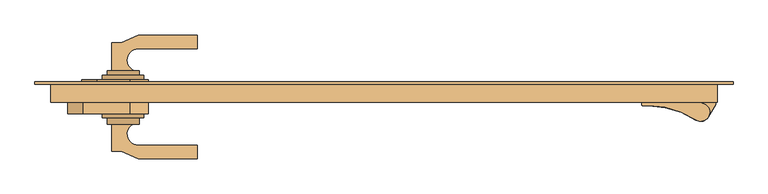
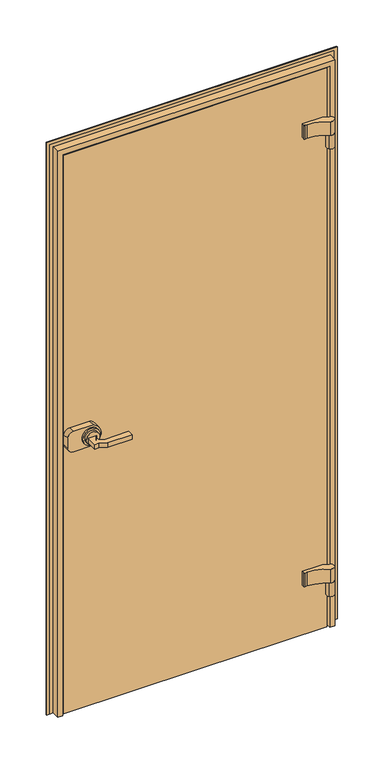
"""IFC4 building model written with IfcOpenShell, lengths in millimetres: door geometry, Doors_Doors_Faraone_Anta : Doors_Doors_Faraone_Anta."""

from ifc_helpers import new_model, si_unit, point, frame, frame_2d, origin, place, context, project, spatial, polyline, circle_curve, trimmed, segment, composite_curve, outline, extrude, faceted_brep, source, transform, mapped, element, save


def door_aa5b3e9e(model_context):
    return source(origin(), model_context, "Body", "SolidModel", [
        extrude(outline(polyline([(371.2008975, 11.599726), (440.9003723, 11.599726), (440.9003723, 1.8997991), (371.2008975, 1.8997991), (371.2008975, 11.599726)])), frame((0.0, 0.0, 1819.0000277), z_axis=(0.0, 0.0, 1.0), x_axis=(1.0, 0.0, 0.0)), (0.0, 0.0, 1.0), 50.0),
        extrude(outline(composite_curve([segment(polyline([(371.2008975, -17.600054), (371.2008975, -8.1001256), (441.2003701, -8.1001256), (441.2003701, -9.6001143), (460.8396194, -16.9560894)]), True, "CONTINUOUS"), segment(trimmed(circle_curve(frame_2d((456.200257, -29.0999673)), 12.9999021), [point((460.8396194, -16.9560894))], [point((449.4124725, -40.1870515))], False, "CARTESIAN"), True, "CONTINUOUS"), segment(trimmed(circle_curve(frame_2d((379.7862865, -147.5843675)), 127.9921454), [point((449.4124725, -40.1870515))], [point((381.2008221, -19.6000389))], True, "CARTESIAN"), True, "CONTINUOUS"), segment(polyline([(381.2008221, -19.6000389), (373.2008824, -19.6000389)]), True, "CONTINUOUS"), segment(trimmed(circle_curve(frame_2d((373.2008824, -17.600054)), 1.9999849), [point((373.2008824, -19.6000389))], [point((371.2008975, -17.600054))], False, "CARTESIAN"), True, "CONTINUOUS")], self_intersect=False)), frame((0.0, 0.0, 1819.0000277), z_axis=(0.0, 0.0, 1.0), x_axis=(1.0, 0.0, 0.0)), (0.0, 0.0, 1.0), 50.0),
        extrude(outline(composite_curve([segment(polyline([(478.0000928, -18.0609582), (467.2229983, -35.9917471)]), True, "CONTINUOUS"), segment(trimmed(circle_curve(frame_2d((456.200257, -29.0999673)), 12.9999021), [point((467.2229983, -35.9917471))], [point((445.8509495, -36.9669419))], False, "CARTESIAN"), True, "CONTINUOUS"), segment(trimmed(circle_curve(frame_2d((456.200257, -29.0999673)), 12.9999021), [point((445.8509495, -36.9669419))], [point((451.8171202, -16.861276))], False, "CARTESIAN"), True, "CONTINUOUS"), segment(polyline([(451.8171202, -16.861276), (456.2037355, -15.0000736), (478.0000928, -15.0000736), (478.0000928, -18.0609582)]), True, "CONTINUOUS")], self_intersect=False)), frame((0.0, 0.0, 1769.0000277), z_axis=(0.0, 0.0, 1.0), x_axis=(1.0, 0.0, 0.0)), (0.0, 0.0, 1.0), 50.0),
        extrude(outline(polyline([(371.2008975, 11.599726), (440.9003723, 11.599726), (440.9003723, 1.8997991), (371.2008975, 1.8997991), (371.2008975, 11.599726)])), frame((0.0, 0.0, 182.0), z_axis=(0.0, 0.0, 1.0), x_axis=(1.0, 0.0, 0.0)), (0.0, 0.0, 1.0), 50.0),
        extrude(outline(composite_curve([segment(polyline([(371.2008975, -17.600054), (371.2008975, -8.1001256), (441.2003701, -8.1001256), (441.2003701, -9.6001143), (460.8396194, -16.9560894)]), True, "CONTINUOUS"), segment(trimmed(circle_curve(frame_2d((456.200257, -29.0999673)), 12.9999021), [point((460.8396194, -16.9560894))], [point((449.4124725, -40.1870515))], False, "CARTESIAN"), True, "CONTINUOUS"), segment(trimmed(circle_curve(frame_2d((379.7862865, -147.5843675)), 127.9921454), [point((449.4124725, -40.1870515))], [point((381.2008221, -19.6000389))], True, "CARTESIAN"), True, "CONTINUOUS"), segment(polyline([(381.2008221, -19.6000389), (373.2008824, -19.6000389)]), True, "CONTINUOUS"), segment(trimmed(circle_curve(frame_2d((373.2008824, -17.600054)), 1.9999849), [point((373.2008824, -19.6000389))], [point((371.2008975, -17.600054))], False, "CARTESIAN"), True, "CONTINUOUS")], self_intersect=False)), frame((0.0, 0.0, 182.0), z_axis=(0.0, 0.0, 1.0), x_axis=(1.0, 0.0, 0.0)), (0.0, 0.0, 1.0), 50.0),
        extrude(outline(composite_curve([segment(polyline([(478.0000928, -18.0609582), (467.2229983, -35.9917471)]), True, "CONTINUOUS"), segment(trimmed(circle_curve(frame_2d((456.200257, -29.0999673)), 12.9999021), [point((467.2229983, -35.9917471))], [point((445.8509495, -36.9669419))], False, "CARTESIAN"), True, "CONTINUOUS"), segment(trimmed(circle_curve(frame_2d((456.200257, -29.0999673)), 12.9999021), [point((445.8509495, -36.9669419))], [point((451.8171202, -16.861276))], False, "CARTESIAN"), True, "CONTINUOUS"), segment(polyline([(451.8171202, -16.861276), (456.2037355, -15.0000736), (478.0000928, -15.0000736), (478.0000928, -18.0609582)]), True, "CONTINUOUS")], self_intersect=False)), frame((0.0, 0.0, 132.0), z_axis=(0.0, 0.0, 1.0), x_axis=(1.0, 0.0, 0.0)), (0.0, 0.0, 1.0), 50.0),
        extrude(outline(composite_curve([segment(trimmed(circle_curve(frame_2d((1003.2884985, -375.8959538)), 23.0897305), [point((1003.2884985, -398.9856843))], [point((1003.2884985, -352.8062233))], False, "CARTESIAN"), True, "CONTINUOUS"), segment(trimmed(circle_curve(frame_2d((1003.2884985, -375.8959538)), 23.0897305), [point((1003.2884985, -352.8062233))], [point((1003.2884985, -398.9856843))], False, "CARTESIAN"), True, "CONTINUOUS")], self_intersect=False)), frame((0.0, -46.355004, 0.0), z_axis=(0.0, 1.0, 0.0), x_axis=(0.0, 0.0, 1.0)), (0.0, 0.0, 1.0), 9.3686894),
        extrude(outline(composite_curve([segment(trimmed(circle_curve(frame_2d((987.7717852, -433.4834563)), 22.4105262), [point((983.5880679, -455.5))], [point((965.361259, -433.4834563))], False, "CARTESIAN"), True, "CONTINUOUS"), segment(polyline([(965.361259, -433.4834563), (965.361259, -368.4834563)]), True, "CONTINUOUS"), segment(trimmed(circle_curve(frame_2d((1002.861259, -378.1489886)), 38.7256054), [point((965.361259, -368.4834563))], [point((1039.5100566, -365.6374682))], False, "CARTESIAN"), True, "CONTINUOUS"), segment(polyline([(1039.5100566, -365.6374682), (1039.5100566, -433.4834563)]), True, "CONTINUOUS"), segment(trimmed(circle_curve(frame_2d((1017.0995304, -433.4834563)), 22.4105262), [point((1039.5100566, -433.4834563))], [point((1021.2832478, -455.5))], False, "CARTESIAN"), True, "CONTINUOUS"), segment(polyline([(1021.2832478, -455.5), (983.5880679, -455.5)]), True, "CONTINUOUS")], self_intersect=False)), frame((0.0, -31.1653283, 0.0), z_axis=(0.0, 1.0, 0.0), x_axis=(0.0, 0.0, 1.0)), (0.0, 0.0, 1.0), 23.0652027),
        extrude(outline(composite_curve([segment(trimmed(circle_curve(frame_2d((987.7717852, -433.4834563)), 22.4105262), [point((983.5880679, -455.5))], [point((965.361259, -433.4834563))], False, "CARTESIAN"), True, "CONTINUOUS"), segment(polyline([(965.361259, -433.4834563), (965.361259, -368.4834563)]), True, "CONTINUOUS"), segment(trimmed(circle_curve(frame_2d((1002.861259, -378.1489886)), 38.7256054), [point((965.361259, -368.4834563))], [point((1039.5100566, -365.6374682))], False, "CARTESIAN"), True, "CONTINUOUS"), segment(polyline([(1039.5100566, -365.6374682), (1039.5100566, -433.4834563)]), True, "CONTINUOUS"), segment(trimmed(circle_curve(frame_2d((1017.0995304, -433.4834563)), 22.4105262), [point((1039.5100566, -433.4834563))], [point((1021.2832478, -455.5))], False, "CARTESIAN"), True, "CONTINUOUS"), segment(polyline([(1021.2832478, -455.5), (983.5880679, -455.5)]), True, "CONTINUOUS")], self_intersect=False)), frame((0.0, -31.1653283, 0.0), z_axis=(0.0, 1.0, 0.0), x_axis=(0.0, 0.0, 1.0)), (0.0, 0.0, 1.0), 23.0652027),
        extrude(outline(composite_curve([segment(trimmed(circle_curve(frame_2d((1003.2884985, -375.8959538)), 30.0), [point((1003.2884985, -405.8959538))], [point((1003.2884985, -345.8959538))], False, "CARTESIAN"), True, "CONTINUOUS"), segment(trimmed(circle_curve(frame_2d((1003.2884985, -375.8959538)), 30.0), [point((1003.2884985, -345.8959538))], [point((1003.2884985, -405.8959538))], False, "CARTESIAN"), True, "CONTINUOUS")], self_intersect=False)), frame((0.0, -36.9863146, 0.0), z_axis=(0.0, 1.0, 0.0), x_axis=(0.0, 0.0, 1.0)), (0.0, 0.0, 1.0), 5.8209863),
        extrude(outline(composite_curve([segment(trimmed(circle_curve(frame_2d((987.7717852, -433.4834563)), 22.4105262), [point((983.5880679, -455.5))], [point((965.361259, -433.4834563))], False, "CARTESIAN"), True, "CONTINUOUS"), segment(polyline([(965.361259, -433.4834563), (965.361259, -368.4834563)]), True, "CONTINUOUS"), segment(trimmed(circle_curve(frame_2d((1002.861259, -378.1489886)), 38.7256054), [point((965.361259, -368.4834563))], [point((1039.5100566, -365.6374682))], False, "CARTESIAN"), True, "CONTINUOUS"), segment(polyline([(1039.5100566, -365.6374682), (1039.5100566, -433.4834563)]), True, "CONTINUOUS"), segment(trimmed(circle_curve(frame_2d((1017.0995304, -433.4834563)), 22.4105262), [point((1039.5100566, -433.4834563))], [point((1021.2832478, -455.5))], False, "CARTESIAN"), True, "CONTINUOUS"), segment(polyline([(1021.2832478, -455.5), (983.5880679, -455.5)]), True, "CONTINUOUS")], self_intersect=False)), frame((0.0, -31.1653283, 0.0), z_axis=(0.0, 1.0, 0.0), x_axis=(0.0, 0.0, 1.0)), (0.0, 0.0, 1.0), 23.0652027),
        extrude(outline(composite_curve([segment(trimmed(circle_curve(frame_2d((1003.2884985, -375.8959538)), 23.0897305), [point((1003.2884985, -398.9856843))], [point((1003.2884985, -352.8062233))], False, "CARTESIAN"), True, "CONTINUOUS"), segment(trimmed(circle_curve(frame_2d((1003.2884985, -375.8959538)), 23.0897305), [point((1003.2884985, -352.8062233))], [point((1003.2884985, -398.9856843))], False, "CARTESIAN"), True, "CONTINUOUS")], self_intersect=False)), frame((0.0, -46.355004, 0.0), z_axis=(0.0, 1.0, 0.0), x_axis=(0.0, 0.0, 1.0)), (0.0, 0.0, 1.0), 14.1896757),
        extrude(outline(composite_curve([segment(trimmed(circle_curve(frame_2d((987.7717852, -433.4834563)), 22.4105262), [point((983.5880679, -455.5))], [point((965.361259, -433.4834563))], False, "CARTESIAN"), True, "CONTINUOUS"), segment(polyline([(965.361259, -433.4834563), (965.361259, -368.4834563)]), True, "CONTINUOUS"), segment(trimmed(circle_curve(frame_2d((1002.861259, -378.1489886)), 38.7256054), [point((965.361259, -368.4834563))], [point((1039.5100566, -365.6374682))], False, "CARTESIAN"), True, "CONTINUOUS"), segment(polyline([(1039.5100566, -365.6374682), (1039.5100566, -433.4834563)]), True, "CONTINUOUS"), segment(trimmed(circle_curve(frame_2d((1017.0995304, -433.4834563)), 22.4105262), [point((1039.5100566, -433.4834563))], [point((1021.2832478, -455.5))], False, "CARTESIAN"), True, "CONTINUOUS"), segment(polyline([(1021.2832478, -455.5), (983.5880679, -455.5)]), True, "CONTINUOUS")], self_intersect=False)), frame((0.0, -31.1653283, 0.0), z_axis=(0.0, 1.0, 0.0), x_axis=(0.0, 0.0, 1.0)), (0.0, 0.0, 1.0), 23.0652027),
        extrude(outline(composite_curve([segment(trimmed(circle_curve(frame_2d((987.7717852, -433.4834563)), 22.4105262), [point((983.5880679, -455.5))], [point((965.361259, -433.4834563))], False, "CARTESIAN"), True, "CONTINUOUS"), segment(polyline([(965.361259, -433.4834563), (965.361259, -368.4834563)]), True, "CONTINUOUS"), segment(trimmed(circle_curve(frame_2d((1002.861259, -378.1489886)), 38.7256054), [point((965.361259, -368.4834563))], [point((1039.5100566, -365.6374682))], False, "CARTESIAN"), True, "CONTINUOUS"), segment(polyline([(1039.5100566, -365.6374682), (1039.5100566, -433.4834563)]), True, "CONTINUOUS"), segment(trimmed(circle_curve(frame_2d((1017.0995304, -433.4834563)), 22.4105262), [point((1039.5100566, -433.4834563))], [point((1021.2832478, -455.5))], False, "CARTESIAN"), True, "CONTINUOUS"), segment(polyline([(1021.2832478, -455.5), (983.5880679, -455.5)]), True, "CONTINUOUS")], self_intersect=False)), frame((0.0, -31.1653283, 0.0), z_axis=(0.0, 1.0, 0.0), x_axis=(0.0, 0.0, 1.0)), (0.0, 0.0, 1.0), 23.0652027),
        extrude(outline(composite_curve([segment(polyline([(-392.3305508, -84.9663543), (-392.3305508, -46.355004), (-362.3717442, -46.355004)]), True, "CONTINUOUS"), segment(trimmed(circle_curve(frame_2d((-354.204395, -60.2485058)), 16.1162956), [point((-362.3717442, -46.355004))], [point((-354.204395, -76.3648014))], True, "CARTESIAN"), True, "CONTINUOUS"), segment(polyline([(-354.204395, -76.3648014), (-269.204395, -76.3648014), (-269.204395, -96.3648014), (-354.204395, -96.3648014), (-378.6484437, -84.9663543), (-392.3305508, -84.9663543)]), True, "CONTINUOUS")], self_intersect=False)), frame((0.0, 0.0, 992.5658854), z_axis=(0.0, 0.0, 1.0), x_axis=(1.0, 0.0, 0.0)), (0.0, 0.0, 1.0), 16.6938628),
        extrude(outline(composite_curve([segment(trimmed(circle_curve(frame_2d((987.7717852, -433.4834563)), 22.4105262), [point((983.5880679, -455.5))], [point((965.361259, -433.4834563))], False, "CARTESIAN"), True, "CONTINUOUS"), segment(polyline([(965.361259, -433.4834563), (965.361259, -368.4834563)]), True, "CONTINUOUS"), segment(trimmed(circle_curve(frame_2d((1002.861259, -378.1489886)), 38.7256054), [point((965.361259, -368.4834563))], [point((1039.5100566, -365.6374682))], False, "CARTESIAN"), True, "CONTINUOUS"), segment(polyline([(1039.5100566, -365.6374682), (1039.5100566, -433.4834563)]), True, "CONTINUOUS"), segment(trimmed(circle_curve(frame_2d((1017.0995304, -433.4834563)), 22.4105262), [point((1039.5100566, -433.4834563))], [point((1021.2832478, -455.5))], False, "CARTESIAN"), True, "CONTINUOUS"), segment(polyline([(1021.2832478, -455.5), (983.5880679, -455.5)]), True, "CONTINUOUS")], self_intersect=False)), frame((0.0, -31.1653283, 0.0), z_axis=(0.0, 1.0, 0.0), x_axis=(0.0, 0.0, 1.0)), (0.0, 0.0, 1.0), 23.0652027),
        extrude(outline(composite_curve([segment(trimmed(circle_curve(frame_2d((1003.2884985, -375.8959538)), 23.0897305), [point((1003.2884985, -398.9856843))], [point((1003.2884985, -352.8062233))], False, "CARTESIAN"), True, "CONTINUOUS"), segment(trimmed(circle_curve(frame_2d((1003.2884985, -375.8959538)), 23.0897305), [point((1003.2884985, -352.8062233))], [point((1003.2884985, -398.9856843))], False, "CARTESIAN"), True, "CONTINUOUS")], self_intersect=False)), frame((0.0, 23.8998744, 0.0), z_axis=(0.0, 1.0, 0.0), x_axis=(0.0, 0.0, 1.0)), (0.0, 0.0, 1.0), 7.0),
        extrude(outline(composite_curve([segment(trimmed(circle_curve(frame_2d((987.7717852, -413.4834563)), 22.4105262), [point((983.5880679, -435.5))], [point((965.361259, -413.4834563))], False, "CARTESIAN"), True, "CONTINUOUS"), segment(polyline([(965.361259, -413.4834563), (965.361259, -368.4834563)]), True, "CONTINUOUS"), segment(trimmed(circle_curve(frame_2d((1002.861259, -378.1489886)), 38.7256054), [point((965.361259, -368.4834563))], [point((1039.5100566, -365.6374682))], False, "CARTESIAN"), True, "CONTINUOUS"), segment(polyline([(1039.5100566, -365.6374682), (1039.5100566, -413.4834563)]), True, "CONTINUOUS"), segment(trimmed(circle_curve(frame_2d((1017.0995304, -413.4834563)), 22.4105262), [point((1039.5100566, -413.4834563))], [point((1021.2832478, -435.5))], False, "CARTESIAN"), True, "CONTINUOUS"), segment(polyline([(1021.2832478, -435.5), (983.5880679, -435.5)]), True, "CONTINUOUS")], self_intersect=False)), frame((0.0, 1.8998744, 0.0), z_axis=(0.0, 1.0, 0.0), x_axis=(0.0, 0.0, 1.0)), (0.0, 0.0, 1.0), 16.0),
        extrude(outline(composite_curve([segment(polyline([(-392.3305508, 70.762087), (-378.6484437, 70.762087), (-354.204395, 82.1605341), (-269.204395, 82.1605341), (-269.204395, 62.1605341), (-354.204395, 62.1605341)]), True, "CONTINUOUS"), segment(trimmed(circle_curve(frame_2d((-354.204395, 46.0442385)), 16.1162956), [point((-354.204395, 62.1605341))], [point((-359.7164928, 30.8998744))], True, "CARTESIAN"), True, "CONTINUOUS"), segment(polyline([(-359.7164928, 30.8998744), (-392.3305508, 30.8998744), (-392.3305508, 70.762087)]), True, "CONTINUOUS")], self_intersect=False)), frame((0.0, 0.0, 992.5658854), z_axis=(0.0, 0.0, 1.0), x_axis=(1.0, 0.0, 0.0)), (0.0, 0.0, 1.0), 16.6938628),
        extrude(outline(composite_curve([segment(trimmed(circle_curve(frame_2d((1003.2884985, -375.8959538)), 30.0), [point((1003.2884985, -405.8959538))], [point((1003.2884985, -345.8959538))], False, "CARTESIAN"), True, "CONTINUOUS"), segment(trimmed(circle_curve(frame_2d((1003.2884985, -375.8959538)), 30.0), [point((1003.2884985, -345.8959538))], [point((1003.2884985, -405.8959538))], False, "CARTESIAN"), True, "CONTINUOUS")], self_intersect=False)), frame((0.0, 17.8998744, 0.0), z_axis=(0.0, 1.0, 0.0), x_axis=(0.0, 0.0, 1.0)), (0.0, 0.0, 1.0), 6.0),
        faceted_brep([(-447.0002625, 14.999774, 0.0), (-447.0002625, 5.9998078, 0.0), (-462.0001619, 5.9998078, 0.0), (-462.0001619, -15.0, 0.0), (-480.0, -15.0, 0.0), (-480.0, 12.9997254, 0.0), (-493.6999352, 12.9997254, 0.0), (-493.6999352, 11.2997382, 0.0), (-502.9998241, 11.2997382, 0.0), (-502.9998241, 14.999774, 0.0), (-447.0002625, 14.999774, 2037.0002901), (-447.0002625, 5.9998078, 2037.0002901), (447.0002625, 5.9998078, 2037.0002901), (447.0002625, 5.9998078, 0.0), (462.0001619, 5.9998078, 0.0), (462.0001619, 5.9998078, 2052.0001896), (-462.0001619, 5.9998078, 2052.0001896), (-462.0001619, -15.0, 2052.0001896), (462.0001619, -15.0, 2052.0001896), (462.0001619, -15.0, 0.0), (480.0, -15.0, 0.0), (480.0, -15.0, 2070.0000277), (-480.0, -15.0, 2070.0000277), (-480.0, 12.9997254, 2070.0000277), (480.0, 12.9997254, 2070.0000277), (480.0, 12.9997254, 0.0), (493.6999352, 12.9997254, 0.0), (493.6999352, 12.9997254, 2083.6999629), (-493.6999352, 12.9997254, 2083.6999629), (-493.6999352, 11.2997382, 2083.6999629), (493.6999352, 11.2997382, 2083.6999629), (493.6999352, 11.2997382, 0.0), (502.9998241, 11.2997382, 0.0), (502.9998241, 11.2997382, 2092.9998518), (-502.9998241, 11.2997382, 2092.9998518), (-502.9998241, 14.999774, 2092.9998518), (502.9998241, 14.999774, 2092.9998518), (502.9998241, 14.999774, 0.0), (447.0002625, 14.999774, 0.0), (447.0002625, 14.999774, 2037.0002901)], [[[0, 1, 2, 3, 4, 5, 6, 7, 8, 9]], [[1, 0, 10, 11]], [[2, 1, 11, 12, 13, 14, 15, 16]], [[3, 2, 16, 17]], [[4, 3, 17, 18, 19, 20, 21, 22]], [[5, 4, 22, 23]], [[6, 5, 23, 24, 25, 26, 27, 28]], [[7, 6, 28, 29]], [[8, 7, 29, 30, 31, 32, 33, 34]], [[9, 8, 34, 35]], [[0, 9, 35, 36, 37, 38, 39, 10]], [[12, 39, 38, 13]], [[38, 37, 32, 31, 26, 25, 20, 19, 14, 13]], [[18, 15, 14, 19]], [[24, 21, 20, 25]], [[30, 27, 26, 31]], [[36, 33, 32, 37]], [[11, 10, 39, 12]], [[17, 16, 15, 18]], [[23, 22, 21, 24]], [[29, 28, 27, 30]], [[35, 34, 33, 36]]]),
        extrude(outline(polyline([(0.0, -455.5), (0.0, 9.5), (0.0, 455.5), (2043.9998511, 455.5), (2043.9998511, -455.5), (0.0, -455.5)])), frame((0.0, -8.1001256, 0.0), z_axis=(0.0, 1.0, 0.0), x_axis=(0.0, 0.0, 1.0)), (0.0, 0.0, 1.0), 10.0),
    ])


if __name__ == "__main__":
    model = new_model("IFC4")
    model_context = context("Model", 3, world=origin())
    ifc_project = project(units=[si_unit("LENGTHUNIT", "METRE", prefix="MILLI")], contexts=[model_context])
    site = spatial("IfcSite", under=ifc_project)
    building = spatial("IfcBuilding", under=site)
    placement = place(None, origin())
    door_shape = door_aa5b3e9e(model_context)
    element("IfcDoor", 1, ObjectType="Doors_Doors_Faraone_Anta : Doors_Doors_Faraone_Anta", at=placement, inside=building, context=model_context, shape_type="MappedRepresentation", body=[
        mapped(door_shape, transform((0.0, 0.0, 0.0), x_axis=(1.0, 0.0, 0.0), y_axis=(0.0, 1.0, 0.0), z_axis=(0.0, 0.0, 1.0))),
    ])
    save(model, "model.ifc")

# Revit data of these elements
# Type "Doors_Doors_Faraone_Anta : Doors_Doors_Faraone_Anta"
#   Type Mark = "58"
#   URL = "https://faraone.it/en/"
#   Product data url = ""
#   Product Guid = ""
#   Model = "Spazio_Anta"
#   Manufacturer = "Faraone"
#   Keynote = "08110"
#   Assembly Code = "C1020100"
#   Analytic Construction = "<None>"
#   Width [instance default] = 1104.999 mm
#   Height [instance default] = 2700 mm
#   Handle Height = 1000 mm
#   Thickness = 11 mm
#   Glass Width [instance default] = 1055.999 mm
#   Middle Hinge [instance default] = yes
#   Edition number = 1
#   Define Thermal Properties by = 1
#   Interior Material = Glass - Faraone - Transparent
#   Handle Type = element 507032
#   Exterior Material = Aluminium - Faraone - Silver
#   Function = (empty or 0)
# Element 1 (IfcDoor, "Doors_Doors_Faraone_Anta : Doors_Doors_Faraone_Anta")
#   Width = 960 mm
#   Height = 2070 mm
#   Glass Width = 911 mm
#   Middle Hinge = no
#   Materials on its faces: "Aluminium - Faraone - Silver", "Glass - Faraone - Transparent"
# Materials
#   "Glass - Faraone - Transparent": class "Glass", colour RGB 0 128 192, transparency 0.9, Description = "Soda Lime Glass", Cost = 0
#   "Aluminium - Faraone - Silver": class "Metal", colour RGB 244 244 244, transparency 0, Description = "Metal - Faraone - Aluminium", Cost = 0
